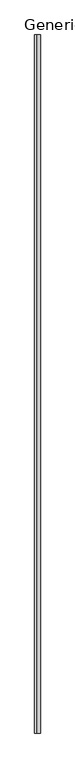
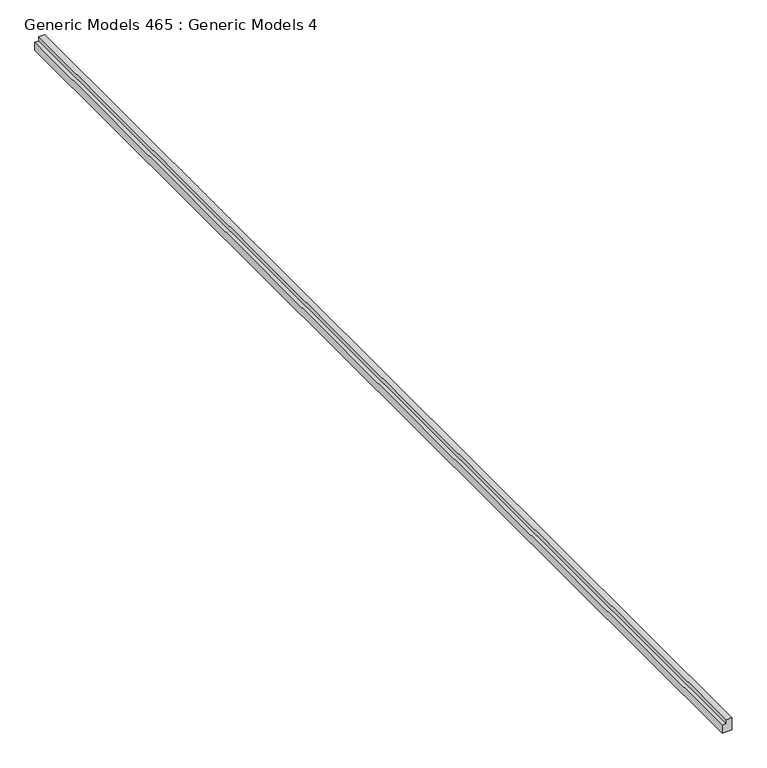
"""IFC4 building model written with IfcOpenShell, lengths in millimetres: proxy geometry, Generic Models 465 : Generic Models 4."""

from ifc_helpers import new_model, si_unit, frame, origin, place, context, project, spatial, polyline, outline, extrude, source, transform, mapped, element, save


def generic_models_465_generic_models_4_7bb24480(model_context):
    return source(origin(), model_context, "Body", "SweptSolid", [
        extrude(outline(polyline([(123291.346, 1727.0263704), (123426.9018649, 1727.0263704), (123426.9018649, 1667.6538533), (123378.2034427, 1667.6538533), (123378.2034427, 1625.4263704), (123291.346, 1625.4263704), (123291.346, 1727.0263704)])), frame((0.0, -5493.3230338, 0.0), z_axis=(0.0, 1.0, 0.0), x_axis=(0.0, 0.0, 1.0)), (0.0, 0.0, 1.0), 12547.6),
    ])


if __name__ == "__main__":
    model = new_model("IFC4")
    model_context = context("Model", 3, world=origin())
    ifc_project = project(units=[si_unit("LENGTHUNIT", "METRE", prefix="MILLI")], contexts=[model_context])
    site = spatial("IfcSite", under=ifc_project)
    building = spatial("IfcBuilding", under=site)
    placement = place(None, origin())
    generic_models_465_generic_models_4_shape = generic_models_465_generic_models_4_7bb24480(model_context)
    element("IfcBuildingElementProxy", 1, Name="Generic Models 465 : Generic Models 4", ObjectType="Generic Models 465 : Generic Models 4", at=placement, inside=building, context=model_context, shape_type="MappedRepresentation", body=[
        mapped(generic_models_465_generic_models_4_shape, transform((0.0, 0.0, 0.0), x_axis=(1.0, 0.0, 0.0), y_axis=(0.0, 1.0, 0.0), z_axis=(0.0, 0.0, 1.0))),
    ])
    save(model, "model.ifc")

# Revit data of these elements
# Element 1 (IfcBuildingElementProxy, "Generic Models 465 : Generic Models 4")
#   Materials on its faces: "_LANDSCAPING STONE T.B.D."
# Materials
#   "_LANDSCAPING STONE T.B.D.": class "Generic", colour RGB 122 131 148, transparency 0, Cost = 0
